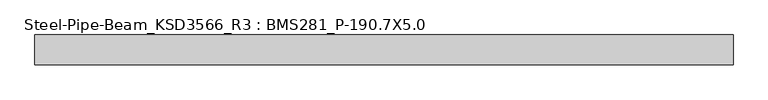
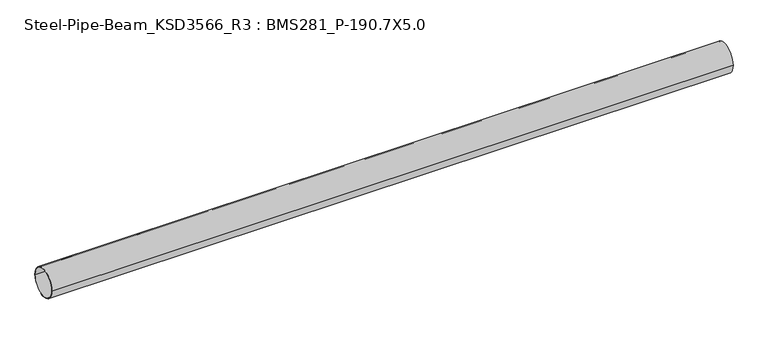
"""IFC4 building model written with IfcOpenShell, lengths in millimetres: member geometry, Steel-Pipe-Beam_KSD3566_R3 : BMS281_P-190.7X5.0."""

from ifc_helpers import new_model, si_unit, point, frame, origin, origin_2d, place, context, project, spatial, circle_curve, trimmed, segment, composite_curve, outline, extrude, source, transform, mapped, element, save


def steel_pipe_beam_ksd3566_r3_bms281_p_190_7x5_0_6e926ad6(model_context):
    return source(origin(), model_context, "Body", "SweptSolid", [
        extrude(outline(composite_curve([segment(trimmed(circle_curve(origin_2d(), 95.35), [point((-95.35, 0.0))], [point((95.35, 0.0))], False, "CARTESIAN"), True, "CONTINUOUS"), segment(trimmed(circle_curve(origin_2d(), 95.35), [point((95.35, 0.0))], [point((-95.35, 0.0))], False, "CARTESIAN"), True, "CONTINUOUS")], self_intersect=False), holes=[composite_curve([segment(trimmed(circle_curve(origin_2d(), 90.35), [point((90.35, 0.0))], [point((-90.35, 0.0))], True, "CARTESIAN"), True, "CONTINUOUS"), segment(trimmed(circle_curve(origin_2d(), 90.35), [point((-90.35, 0.0))], [point((90.35, 0.0))], True, "CARTESIAN"), True, "CONTINUOUS")], self_intersect=False)]), frame((-2233.2484247, 0.0, 0.0), z_axis=(1.0, 0.0, 0.0), x_axis=(0.0, 1.0, 0.0)), (0.0, 0.0, 1.0), 4448.4931366),
    ])


if __name__ == "__main__":
    model = new_model("IFC4")
    model_context = context("Model", 3, world=origin())
    ifc_project = project(units=[si_unit("LENGTHUNIT", "METRE", prefix="MILLI")], contexts=[model_context])
    site = spatial("IfcSite", under=ifc_project)
    building = spatial("IfcBuilding", under=site)
    placement = place(None, origin())
    steel_pipe_beam_ksd3566_r3_bms281_p_190_7x5_0_shape = steel_pipe_beam_ksd3566_r3_bms281_p_190_7x5_0_6e926ad6(model_context)
    element("IfcMember", 1, ObjectType="Steel-Pipe-Beam_KSD3566_R3 : BMS281_P-190.7X5.0", at=placement, inside=building, context=model_context, shape_type="MappedRepresentation", body=[
        mapped(steel_pipe_beam_ksd3566_r3_bms281_p_190_7x5_0_shape, transform((0.0, 0.0, 0.0), x_axis=(1.0, 0.0, 0.0), y_axis=(0.0, 1.0, 0.0), z_axis=(0.0, 0.0, 1.0))),
    ])
    save(model, "model.ifc")

# Revit data of these elements
# Type "Steel-Pipe-Beam_KSD3566_R3 : BMS281_P-190.7X5.0"
#   Keynote = "P-190.7X5.0"
#   SteelWeight = "Light"
#   t = 0.0050 m
#   Surface Area = 0.599102 m²/m
#   Section Area = 29.1697 cm²
#   Mass per Unit Length = 22.8982 kg/m
#   Length [instance default] = 1.5000 m
#   D = 0.1907 m
#   hec_material4 [instance default] = none
#   hec_material3 [instance default] = none
#   hec_material2 [instance default] = none
#   hec_material1 [instance default] = none
#   Structural Material [instance default] = Steel, 45-345
#   Assembly Code = ""
# Element 1 (IfcMember, "Steel-Pipe-Beam_KSD3566_R3 : BMS281_P-190.7X5.0")
#   Structural Material = none
# Materials
#   "Steel, 45-345": class "Metal", colour RGB 189 187 185, transparency 0, Description = "Steel 345 MPa", Cost = 0
